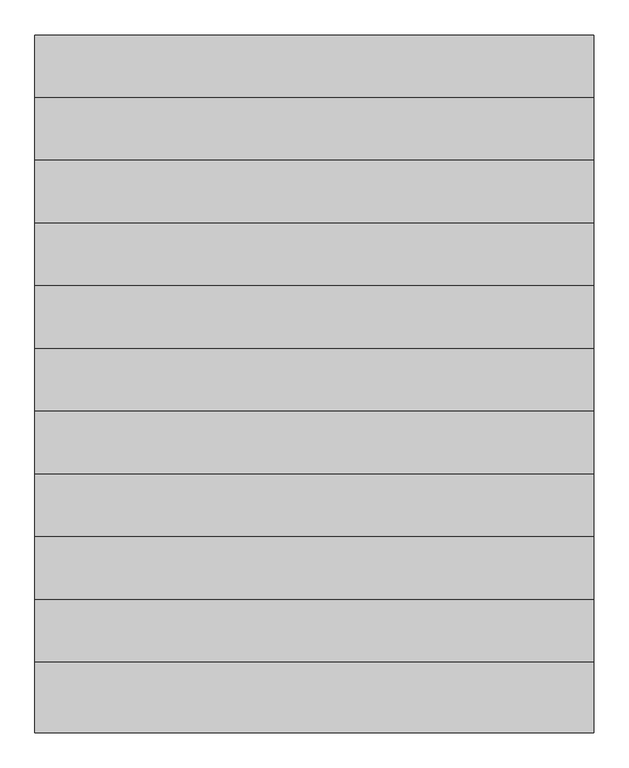
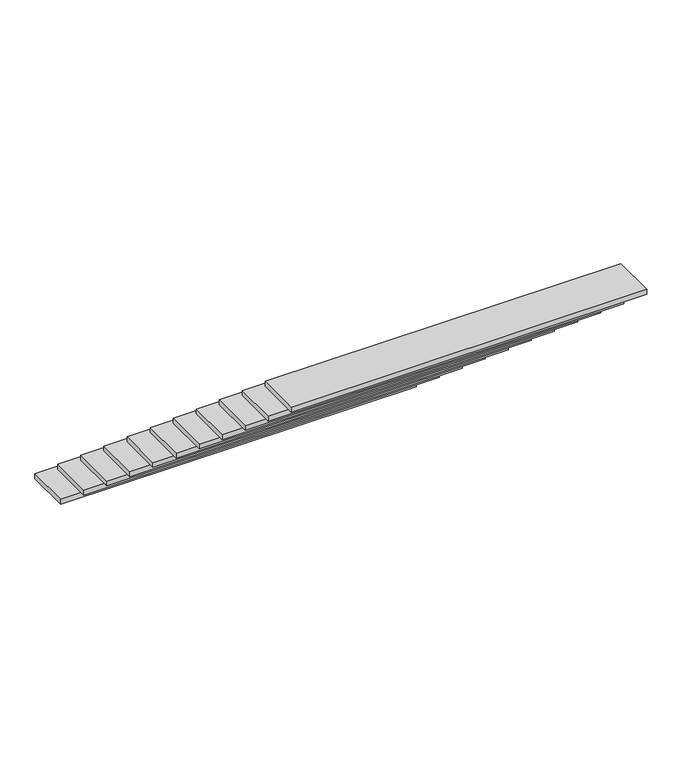
"""IFC4 building model written with IfcOpenShell, lengths in millimetres: stair flight geometry."""

from ifc_helpers import new_model, si_unit, frame, origin, origin_with_axes, place, context, project, spatial, polyline, outline, extrude, source, transform, mapped, element, save


def stair_flight_bf35e301(model_context):
    return source(origin(), model_context, "Body", "SweptSolid", [
        extrude(outline(polyline([(8467.9494269, 8638.7618365), (6373.7670994, 8638.7618365), (6373.7670994, 8903.7618365), (8467.9494269, 8903.7618365), (8467.9494269, 8638.7618365)])), frame((0.0, 0.0, -1400.0), z_axis=(0.0, 0.0, 1.0), x_axis=(1.0, 0.0, 0.0)), (0.0, 0.0, 1.0), 30.0),
        extrude(outline(polyline([(8467.9494269, 8403.7618365), (6373.7670994, 8403.7618365), (6373.7670994, 8668.7618365), (8467.9494269, 8668.7618365), (8467.9494269, 8403.7618365)])), frame((0.0, 0.0, -1200.0), z_axis=(0.0, 0.0, 1.0), x_axis=(1.0, 0.0, 0.0)), (0.0, 0.0, 1.0), 30.0),
        extrude(outline(polyline([(8467.9494269, 8168.7618365), (6373.7670994, 8168.7618365), (6373.7670994, 8433.7618365), (8467.9494269, 8433.7618365), (8467.9494269, 8168.7618365)])), frame((0.0, 0.0, -1000.0), z_axis=(0.0, 0.0, 1.0), x_axis=(1.0, 0.0, 0.0)), (0.0, 0.0, 1.0), 30.0),
        extrude(outline(polyline([(8467.9494269, 7933.7618365), (6373.7670994, 7933.7618365), (6373.7670994, 8198.7618365), (8467.9494269, 8198.7618365), (8467.9494269, 7933.7618365)])), frame((0.0, 0.0, -800.0), z_axis=(0.0, 0.0, 1.0), x_axis=(1.0, 0.0, 0.0)), (0.0, 0.0, 1.0), 30.0),
        extrude(outline(polyline([(8467.9494269, 7698.7618365), (6373.7670994, 7698.7618365), (6373.7670994, 7963.7618365), (8467.9494269, 7963.7618365), (8467.9494269, 7698.7618365)])), frame((0.0, 0.0, -600.0), z_axis=(0.0, 0.0, 1.0), x_axis=(1.0, 0.0, 0.0)), (0.0, 0.0, 1.0), 30.0),
        extrude(outline(polyline([(8467.9494269, 7463.7618365), (6373.7670994, 7463.7618365), (6373.7670994, 7728.7618365), (8467.9494269, 7728.7618365), (8467.9494269, 7463.7618365)])), frame((0.0, 0.0, -400.0), z_axis=(0.0, 0.0, 1.0), x_axis=(1.0, 0.0, 0.0)), (0.0, 0.0, 1.0), 30.0),
        extrude(outline(polyline([(8467.9494269, 7228.7618365), (6373.7670994, 7228.7618365), (6373.7670994, 7493.7618365), (8467.9494269, 7493.7618365), (8467.9494269, 7228.7618365)])), frame((0.0, 0.0, -200.0), z_axis=(0.0, 0.0, 1.0), x_axis=(1.0, 0.0, 0.0)), (0.0, 0.0, 1.0), 30.0),
        extrude(outline(polyline([(8467.9494269, 6993.7618365), (6373.7670994, 6993.7618365), (6373.7670994, 7258.7618365), (8467.9494269, 7258.7618365), (8467.9494269, 6993.7618365)])), origin_with_axes(), (0.0, 0.0, 1.0), 30.0),
        extrude(outline(polyline([(8467.9494269, 6758.7618365), (6373.7670994, 6758.7618365), (6373.7670994, 7023.7618365), (8467.9494269, 7023.7618365), (8467.9494269, 6758.7618365)])), frame((0.0, 0.0, 200.0), z_axis=(0.0, 0.0, 1.0), x_axis=(1.0, 0.0, 0.0)), (0.0, 0.0, 1.0), 30.0),
        extrude(outline(polyline([(8467.9494269, 6523.7618365), (6373.7670994, 6523.7618365), (6373.7670994, 6788.7618365), (8467.9494269, 6788.7618365), (8467.9494269, 6523.7618365)])), frame((0.0, 0.0, 400.0), z_axis=(0.0, 0.0, 1.0), x_axis=(1.0, 0.0, 0.0)), (0.0, 0.0, 1.0), 30.0),
        extrude(outline(polyline([(8467.9494269, 6288.7618365), (6373.7670994, 6288.7618365), (6373.7670994, 6553.7618365), (8467.9494269, 6553.7618365), (8467.9494269, 6288.7618365)])), frame((0.0, 0.0, 600.0), z_axis=(0.0, 0.0, 1.0), x_axis=(1.0, 0.0, 0.0)), (0.0, 0.0, 1.0), 30.0),
    ])


if __name__ == "__main__":
    model = new_model("IFC4")
    model_context = context("Model", 3, world=origin())
    ifc_project = project(units=[si_unit("LENGTHUNIT", "METRE", prefix="MILLI")], contexts=[model_context])
    site = spatial("IfcSite", under=ifc_project)
    building = spatial("IfcBuilding", under=site)
    placement = place(None, origin())
    stair_flight_shape = stair_flight_bf35e301(model_context)
    element("IfcStairFlight", 1, at=placement, inside=building, context=model_context, shape_type="MappedRepresentation", body=[
        mapped(stair_flight_shape, transform((0.0, 0.0, 0.0), x_axis=(1.0, 0.0, 0.0), y_axis=(0.0, 1.0, 0.0), z_axis=(0.0, 0.0, 1.0))),
    ])
    save(model, "model.ifc")

# Revit data of these elements
# Element 1 (IfcStairFlight)
#   Materials on its faces: "Stahlbeton - Sichtbeton (2)"
# Materials
#   "Stahlbeton - Sichtbeton (2)": class "Beton", colour RGB 192 192 192, transparency 0, Cost = 0
